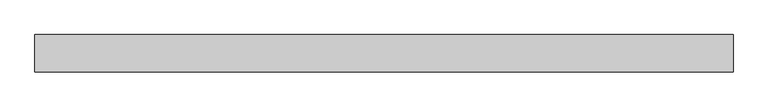
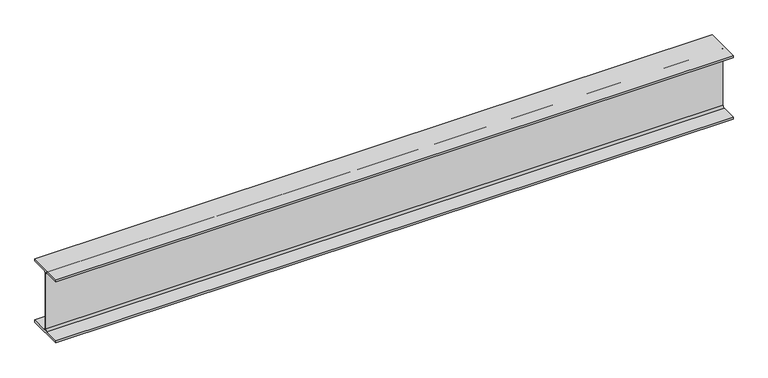
"""IFC4 building model written with IfcOpenShell, lengths in millimetres: beam geometry, Steel Beam_H-KSD3502 : H_SB_ASB_H-200x200x8x12."""

from ifc_helpers import new_model, si_unit, point, frame, frame_2d, origin, place, context, project, spatial, polyline, circle_curve, trimmed, segment, composite_curve, outline, extrude, source, transform, mapped, element, save


def beam_2c81aa5d(model_context):
    return source(origin(), model_context, "Body", "SweptSolid", [
        extrude(outline(composite_curve([segment(polyline([(82.5, -141.5), (82.5, -151.7), (-82.5, -151.7), (-82.5, -141.5), (-11.9, -141.5)]), True, "CONTINUOUS"), segment(trimmed(circle_curve(frame_2d((-11.9, -132.6)), 8.9), [point((-11.9, -141.5))], [point((-3.0, -132.6))], True, "CARTESIAN"), True, "CONTINUOUS"), segment(polyline([(-3.0, -132.6), (-3.0, 132.6)]), True, "CONTINUOUS"), segment(trimmed(circle_curve(frame_2d((-11.9, 132.6)), 8.9), [point((-3.0, 132.6))], [point((-11.9, 141.5))], True, "CARTESIAN"), True, "CONTINUOUS"), segment(polyline([(-11.9, 141.5), (-82.5, 141.5), (-82.5, 151.7), (82.5, 151.7), (82.5, 141.5), (11.9, 141.5)]), True, "CONTINUOUS"), segment(trimmed(circle_curve(frame_2d((11.9, 132.6)), 8.9), [point((11.9, 141.5))], [point((3.0, 132.6))], True, "CARTESIAN"), True, "CONTINUOUS"), segment(polyline([(3.0, 132.6), (3.0, -132.6)]), True, "CONTINUOUS"), segment(trimmed(circle_curve(frame_2d((11.9, -132.6)), 8.9), [point((3.0, -132.6))], [point((11.9, -141.5))], True, "CARTESIAN"), True, "CONTINUOUS"), segment(polyline([(11.9, -141.5), (82.5, -141.5)]), True, "CONTINUOUS")], self_intersect=False)), frame((-1489.1986147, 0.0, 0.0), z_axis=(1.0, 0.0, 0.0), x_axis=(0.0, 1.0, 0.0)), (0.0, 0.0, 1.0), 3067.173634),
    ])


if __name__ == "__main__":
    model = new_model("IFC4")
    model_context = context("Model", 3, world=origin())
    ifc_project = project(units=[si_unit("LENGTHUNIT", "METRE", prefix="MILLI")], contexts=[model_context])
    site = spatial("IfcSite", under=ifc_project)
    building = spatial("IfcBuilding", under=site)
    placement = place(None, origin())
    beam_shape = beam_2c81aa5d(model_context)
    element("IfcBeam", 1, ObjectType="Steel Beam_H-KSD3502 : H_SB_ASB_H-200x200x8x12", at=placement, inside=building, context=model_context, shape_type="MappedRepresentation", body=[
        mapped(beam_shape, transform((0.0, 0.0, 0.0), x_axis=(1.0, 0.0, 0.0), y_axis=(0.0, 1.0, 0.0), z_axis=(0.0, 0.0, 1.0))),
    ])
    save(model, "model.ifc")

# Revit data of these elements
# Type "Steel Beam_H-KSD3502 : H_SB_ASB_H-200x200x8x12"
#   Width = 20.0 cm
#   Web Thickness = 0.8 cm
#   Web Fillet = 1.3 cm
#   Warping Constant = 141376.0 cm⁶
#   Torsional Moment of Inertia = 26.2485 cm⁴
#   Torsional Modulus = 1.0 cm³
#   Section Area = 63.53 cm²
#   Plastic Modulus weak axis = 244.0 cm³
#   Plastic Modulus strong axis = 525.0 cm³
#   Perimeter = 1.16 m²/m
#   Nominal Weight = 49.90 kgf/m
#   Moment of Inertia weak axis = 1600.00 cm⁴
#   Moment of Inertia strong axis = 4720.00 cm⁴
#   Height = 20.0 cm
#   Flange Thickness = 1.2 cm
#   Elastic Modulus weak axis = 160.0 cm³
#   Elastic Modulus strong axis = 472.0 cm³
#   Centroid Vertical = 10.0 cm
#   Centroid Horizontal = 10.0 cm
#   Length [instance default] = 1.5240 m
#   Structural Material [instance default] = Steel, 45-345
#   Assembly Code = ""
# Element 1 (IfcBeam, "Steel Beam_H-KSD3502 : H_SB_ASB_H-200x200x8x12")
#   Structural Material = none
# Materials
#   "Steel, 45-345": class "Metal", colour RGB 189 187 185, transparency 0, Description = "Steel 345 MPa", Cost = 0
